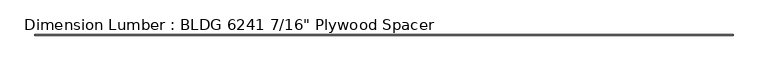
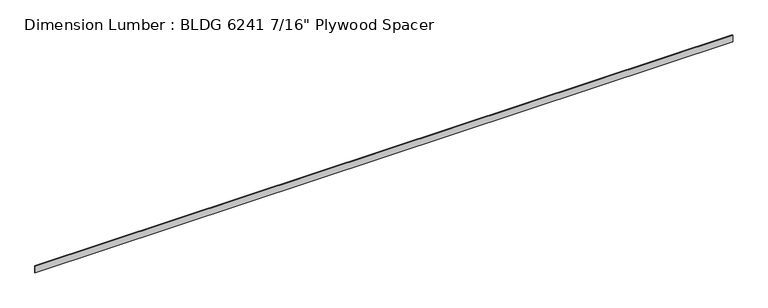
"""IFC4 building model written with IfcOpenShell, lengths in millimetres: beam geometry."""

import ifcopenshell
import ifcopenshell.guid

model = None  # the IFC model being written
_history = None  # IfcOwnerHistory: only IFC2X3 demands one
_inside = {}  # id of a spatial element -> (the spatial element, [elements in it])
_under = {}  # id of a project, library or spatial element -> (it, [spatial elements below it])
_declared = {}  # id of a project -> (the project, [libraries it declares])
_typed = {}  # id of a type object -> (the type object, [elements of that type])
_made_of = {}  # id of a material, layer set ... -> (it, [elements and type objects made of it])


def new_model(schema):
    """Start an empty IFC model of exactly this schema.

    Asked for "IFC4X3", IfcOpenShell would pick the latest addendum, in which some entities
    have other attributes; the version numbers below select the first issue.
    IFC2X3 requires an IfcOwnerHistory on every rooted entity: one is made here for all.
    """
    global model, _history
    if schema == "IFC4X3":
        model = ifcopenshell.file(schema_version=(4, 3, 0, 0))
    else:
        model = ifcopenshell.file(schema=schema)
    _inside.clear()
    _under.clear()
    _declared.clear()
    _typed.clear()
    _made_of.clear()
    _history = None
    if model.schema == "IFC2X3":
        org = make("IfcOrganization", Name="unknown")
        user = make(
            "IfcPersonAndOrganization",
            ThePerson=make("IfcPerson", FamilyName="unknown"),
            TheOrganization=org,
        )
        app = make(
            "IfcApplication",
            ApplicationDeveloper=org,
            Version="unknown",
            ApplicationFullName="unknown",
            ApplicationIdentifier="unknown",
        )
        _history = make(
            "IfcOwnerHistory",
            OwningUser=user,
            OwningApplication=app,
            ChangeAction="ADDED",
            CreationDate=0,
        )
    return model


def make(cls, **values):
    """One entity of the class cls with the attributes given. An attribute that is None is left unset."""
    return model.create_entity(
        cls, **{name: value for name, value in values.items() if value is not None}
    )


def rooted(cls, **values):
    """An entity with a GlobalId (a new one), such as an element, a storey or a relation."""
    return make(cls, GlobalId=ifcopenshell.guid.new(), OwnerHistory=_history, **values)


def si_unit(unit_type, name, prefix=None):
    """IfcSIUnit, for example si_unit("LENGTHUNIT", "METRE", prefix="MILLI")."""
    return make("IfcSIUnit", UnitType=unit_type, Prefix=prefix, Name=name)


def assignment(units):
    """IfcUnitAssignment: the units of a project."""
    return None if units is None else make("IfcUnitAssignment", Units=units)


def point(xyz):
    """IfcCartesianPoint."""
    return None if xyz is None else make("IfcCartesianPoint", Coordinates=xyz)


def direction(xyz):
    """IfcDirection."""
    return None if xyz is None else make("IfcDirection", DirectionRatios=xyz)


def frame(location, z_axis=None, x_axis=None):
    """IfcAxis2Placement3D, a coordinate frame: its origin and axes. An axis left out is left unset."""
    return make(
        "IfcAxis2Placement3D",
        Location=point(location),
        Axis=direction(z_axis),
        RefDirection=direction(x_axis),
    )


def origin():
    """The frame at (0, 0, 0) with its axes left unset."""
    return frame((0.0, 0.0, 0.0))


def place(relative_to, where):
    """IfcLocalPlacement: puts the frame where relative to a parent placement (None: the world)."""
    return make(
        "IfcLocalPlacement", PlacementRelTo=relative_to, RelativePlacement=where
    )


def context(
    kind, dimensions, precision=None, world=None, true_north=None, identifier=None
):
    """IfcGeometricRepresentationContext, for example the 3D "Model" context."""
    return make(
        "IfcGeometricRepresentationContext",
        ContextIdentifier=identifier,
        ContextType=kind,
        CoordinateSpaceDimension=dimensions,
        Precision=precision,
        WorldCoordinateSystem=world,
        TrueNorth=true_north,
    )


def project(units=None, contexts=None):
    """IfcProject with its units and contexts."""
    return rooted(
        "IfcProject",
        Name="project",
        RepresentationContexts=contexts,
        UnitsInContext=assignment(units),
    )


def spatial(cls, under=None, at=None, **own):
    """A site, building, storey or space (cls), placed at a placement, below another one or the project."""
    s = rooted(cls, ObjectPlacement=at, **own)
    if under is not None:
        _under.setdefault(under.id(), (under, []))[1].append(s)
    return s


def polyline(points):
    """IfcPolyline through the points."""
    return make("IfcPolyline", Points=[point(p) for p in points])


def outline(outer, holes=None, kind="AREA"):
    """IfcArbitraryClosedProfileDef: a profile drawn as a closed curve; with holes, ...WithVoids."""
    if holes is None:
        return make("IfcArbitraryClosedProfileDef", ProfileType=kind, OuterCurve=outer)
    return make(
        "IfcArbitraryProfileDefWithVoids",
        ProfileType=kind,
        OuterCurve=outer,
        InnerCurves=holes,
    )


def extrude(swept, where, along, depth):
    """IfcExtrudedAreaSolid: the profile swept, set in the frame where, extruded along a direction by depth."""
    return make(
        "IfcExtrudedAreaSolid",
        SweptArea=swept,
        Position=where,
        ExtrudedDirection=direction(along),
        Depth=depth,
    )


def shape(context_of_items, identifier, shape_type, items):
    """IfcShapeRepresentation: the items that make up one representation, for example the "Body"."""
    return make(
        "IfcShapeRepresentation",
        ContextOfItems=context_of_items,
        RepresentationIdentifier=identifier,
        RepresentationType=shape_type,
        Items=items,
    )


def source(mapping_origin, context_of_items, identifier, shape_type, items):
    """IfcRepresentationMap: a shape defined once, which mapped items show again and again."""
    return make(
        "IfcRepresentationMap",
        MappingOrigin=mapping_origin,
        MappedRepresentation=shape(context_of_items, identifier, shape_type, items),
    )


def transform(
    local_origin,
    x_axis=None,
    y_axis=None,
    z_axis=None,
    scale=None,
    scale2=None,
    scale3=None,
    uniform=True,
):
    """IfcCartesianTransformationOperator3D, or its non-uniform kind. x_axis, y_axis, z_axis: its Axis1, 2, 3."""
    if uniform:
        return make(
            "IfcCartesianTransformationOperator3D",
            Axis1=direction(x_axis),
            Axis2=direction(y_axis),
            LocalOrigin=point(local_origin),
            Scale=scale,
            Axis3=direction(z_axis),
        )
    return make(
        "IfcCartesianTransformationOperator3DnonUniform",
        Axis1=direction(x_axis),
        Axis2=direction(y_axis),
        LocalOrigin=point(local_origin),
        Scale=scale,
        Axis3=direction(z_axis),
        Scale2=scale2,
        Scale3=scale3,
    )


def mapped(mapping_source, mapping_target):
    """IfcMappedItem: shows the shape of a source again, moved by a transform."""
    return make(
        "IfcMappedItem", MappingSource=mapping_source, MappingTarget=mapping_target
    )


def made_of(thing, what):
    """Note that an element or type object is made of a material, layer set ...; save() writes the relation."""
    if what is not None:
        _made_of.setdefault(what.id(), (what, []))[1].append(thing)
    return thing


def element(
    cls,
    number,
    at=None,
    inside=None,
    cuts=None,
    type_object=None,
    material=None,
    context=None,
    identifier="Body",
    shape_type=None,
    held_by="IfcProductDefinitionShape",
    body=None,
    shapes=None,
    **own,
):
    """One element of the class cls, such as IfcWall. Its Tag is "e" and its number.

    at: its placement. inside: the storey or other place that contains it. cuts: it is an
    opening in that element (IfcRelVoidsElement). A single representation is given by context,
    identifier, shape_type and body (its items); several are given by shapes. held_by: the class
    of the entity that holds the representations. save() writes the other relations.
    """
    e = rooted(cls, Tag="e%d" % number, ObjectPlacement=at, **own)
    if body is not None:
        shapes = [shape(context, identifier, shape_type, body)]
    if shapes is not None:
        e.Representation = make(held_by, Representations=shapes)
    if inside is not None:
        _inside.setdefault(inside.id(), (inside, []))[1].append(e)
    if cuts is not None:
        rooted(
            "IfcRelVoidsElement", RelatingBuildingElement=cuts, RelatedOpeningElement=e
        )
    if type_object is not None:
        _typed.setdefault(type_object.id(), (type_object, []))[1].append(e)
    return made_of(e, material)


def aggregate(whole, parts):
    """IfcRelAggregates: a whole, such as a stair, and the parts it consists of."""
    return rooted("IfcRelAggregates", RelatingObject=whole, RelatedObjects=parts)


def save(model, path):
    """Write the relations noted so far, then the file.

    IfcRelAggregates (storeys below a building ...), IfcRelContainedInSpatialStructure (elements
    in a storey), IfcRelDefinesByType, IfcRelAssociatesMaterial and IfcRelDeclares: one each for
    every whole, place, type object, material and project.
    """
    for whole, parts in _under.values():
        aggregate(whole, parts)
    for where, things in _inside.values():
        rooted(
            "IfcRelContainedInSpatialStructure",
            RelatedElements=things,
            RelatingStructure=where,
        )
    for kind, things in _typed.values():
        rooted("IfcRelDefinesByType", RelatedObjects=things, RelatingType=kind)
    for what, things in _made_of.values():
        rooted("IfcRelAssociatesMaterial", RelatedObjects=things, RelatingMaterial=what)
    for by, libraries in _declared.values():
        rooted("IfcRelDeclares", RelatingContext=by, RelatedDefinitions=libraries)
    model.write(path)


def beam_af2566d3(model_context):
    return source(origin(), model_context, "Body", "SweptSolid", [
        extrude(outline(polyline([(6458.3020508, 5.55625), (6458.3020508, -5.55625), (-6159.1479492, -5.55625), (-6159.1479492, 5.55625), (6458.3020508, 5.55625)])), frame((0.0, 0.0, -63.5), z_axis=(0.0, 0.0, 1.0), x_axis=(1.0, 0.0, 0.0)), (0.0, 0.0, 1.0), 127.0),
    ])


if __name__ == "__main__":
    model = new_model("IFC4")
    model_context = context("Model", 3, world=origin())
    ifc_project = project(units=[si_unit("LENGTHUNIT", "METRE", prefix="MILLI")], contexts=[model_context])
    site = spatial("IfcSite", under=ifc_project)
    building = spatial("IfcBuilding", under=site)
    placement = place(None, origin())
    beam_shape = beam_af2566d3(model_context)
    element("IfcBeam", 1, ObjectType="Dimension Lumber : BLDG 6241 7/16\" Plywood Spacer", at=placement, inside=building, context=model_context, shape_type="MappedRepresentation", body=[
        mapped(beam_shape, transform((0.0, 0.0, 0.0), x_axis=(1.0, 0.0, 0.0), y_axis=(0.0, 1.0, 0.0), z_axis=(0.0, 0.0, 1.0))),
    ])
    save(model, "model.ifc")

# Revit data of these elements
# Type "Dimension Lumber : BLDG 6241 7/16\" Plywood Spacer"
#   Assembly Code = "B10"
#   A = 0.273472 SF
#   Length [instance default] = 5' - 0"
#   b = 0' - 0 7/16"
#   d = 0' - 5"
#   Structural Material [instance default] = Softwood, Lumber
# Element 1 (IfcBeam, "Dimension Lumber : BLDG 6241 7/16\" Plywood Spacer")
#   Structural Material = Plywood, Sheathing
#   Materials on its faces: "Plywood, Sheathing"
# Materials
#   "Softwood, Lumber": class "Wood", colour RGB 223 192 134, transparency 0, Description = "Pinus Echinata", Cost = 0
#   "Plywood, Sheathing": class "Wood", colour RGB 212 179 113, transparency 0, Description = "Plywood, sheathing grade", Cost = 0
